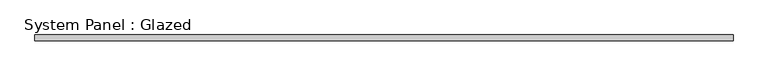
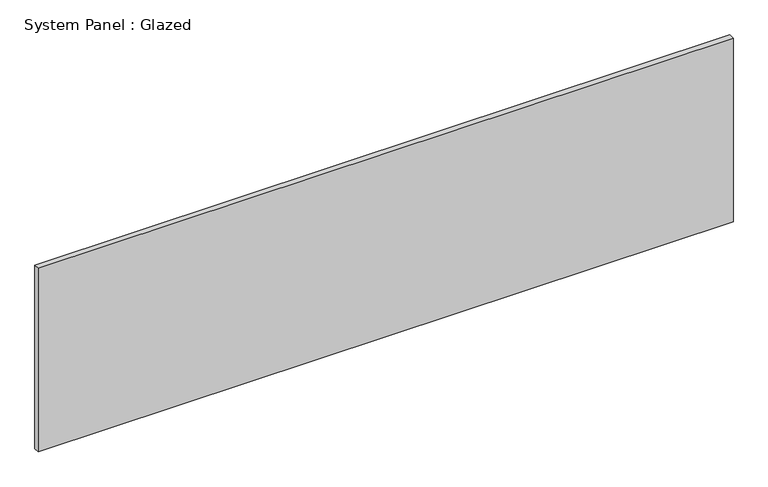
"""IFC4 building model written with IfcOpenShell, lengths in millimetres: plate geometry, System Panel : Glazed."""

from ifc_helpers import new_model, si_unit, origin, origin_with_axes, place, context, project, spatial, polyline, outline, extrude, source, transform, mapped, element, save


def system_panel_glazed_495097d9(model_context):
    return source(origin(), model_context, "Body", "SweptSolid", [
        extrude(outline(polyline([(1549.4, -44.45), (-1549.4, -44.45), (-1549.4, -19.05), (1549.4, -19.05), (1549.4, -44.45)])), origin_with_axes(), (0.0, 0.0, 1.0), 866.081558),
    ])


if __name__ == "__main__":
    model = new_model("IFC4")
    model_context = context("Model", 3, world=origin())
    ifc_project = project(units=[si_unit("LENGTHUNIT", "METRE", prefix="MILLI")], contexts=[model_context])
    site = spatial("IfcSite", under=ifc_project)
    building = spatial("IfcBuilding", under=site)
    placement = place(None, origin())
    system_panel_glazed_shape = system_panel_glazed_495097d9(model_context)
    element("IfcPlate", 1, ObjectType="System Panel : Glazed", at=placement, inside=building, context=model_context, shape_type="MappedRepresentation", body=[
        mapped(system_panel_glazed_shape, transform((0.0, 0.0, 0.0), x_axis=(1.0, 0.0, 0.0), y_axis=(0.0, 1.0, 0.0), z_axis=(0.0, 0.0, 1.0))),
    ])
    save(model, "model.ifc")

# Revit data of these elements
# Type "System Panel : Glazed"
#   Construction Type Id = "GSP4R"
#   Analytic Construction = "1/8 in Pilkington single glazing"
#   Visual Light Transmittance = 0.9
#   Solar Heat Gain Coefficient = 0.86
#   Heat Transfer Coefficient (U) = 1.18115 BTU/(h·ft²·°F)
#   Define Thermal Properties by = 1
# Element 1 (IfcPlate, "System Panel : Glazed")
#   Materials on its faces: "Glass"
# Materials
#   "Glass": class "Glass", colour RGB 0 128 192, transparency 0.75, Description = "Soda Lime Glass", Cost = 0
